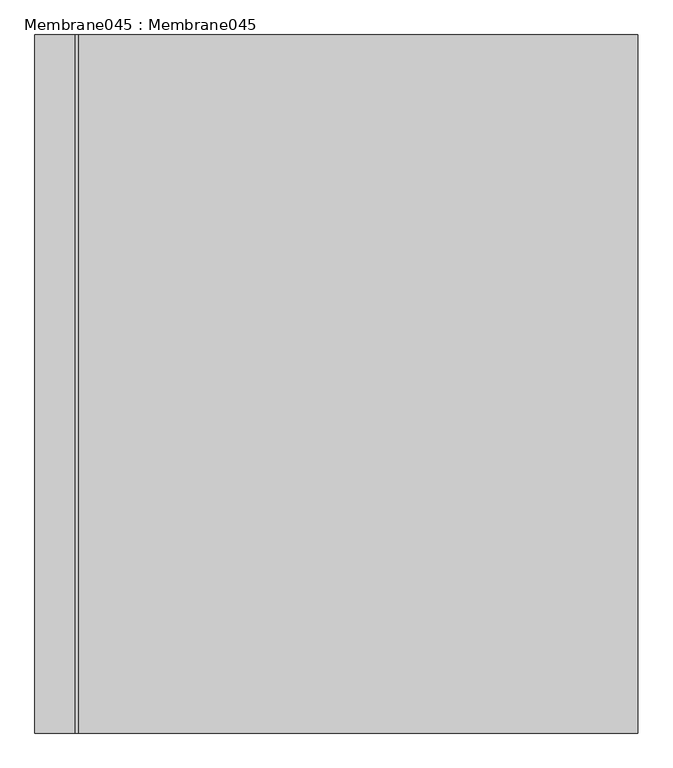
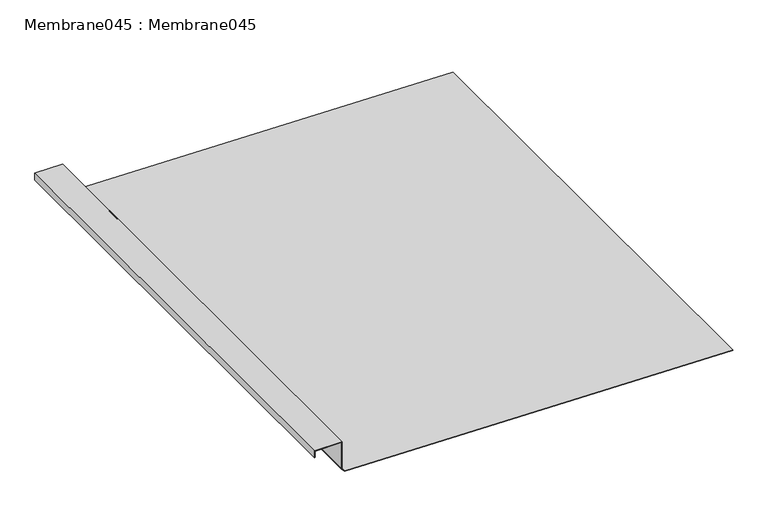
"""IFC4 building model written with IfcOpenShell, lengths in millimetres: proxy geometry, Membrane045 : Membrane045."""

from ifc_helpers import new_model, si_unit, frame, origin, place, context, project, spatial, polyline, outline, extrude, source, transform, mapped, element, save


def membrane045_membrane045_dc4fe3ef(model_context):
    return source(origin(), model_context, "Body", "SweptSolid", [
        extrude(outline(polyline([(40136.1757812, -7230.3012695), (40136.1757812, -7228.3012695), (40163.4960083, -7228.3012695), (40163.4960083, -7118.3154297), (40045.8515625, -7118.3154297), (40034.453125, -7107.1005859), (40000.937504, -5503.7121051), (40002.9370672, -5503.6703083), (40036.4356875, -7106.2454745), (40046.6704939, -7116.3154297), (40165.4960083, -7116.3154297), (40165.4960083, -7230.3012695), (40136.1757812, -7230.3012695)])), frame((0.0, 7982.1531721, 0.0), z_axis=(0.0, 1.0, 0.0), x_axis=(0.0, 0.0, 1.0)), (0.0, 0.0, 1.0), 2000.0),
    ])


if __name__ == "__main__":
    model = new_model("IFC4")
    model_context = context("Model", 3, world=origin())
    ifc_project = project(units=[si_unit("LENGTHUNIT", "METRE", prefix="MILLI")], contexts=[model_context])
    site = spatial("IfcSite", under=ifc_project)
    building = spatial("IfcBuilding", under=site)
    placement = place(None, origin())
    membrane045_membrane045_shape = membrane045_membrane045_dc4fe3ef(model_context)
    element("IfcBuildingElementProxy", 1, Name="Membrane045 : Membrane045", ObjectType="Membrane045 : Membrane045", at=placement, inside=building, context=model_context, shape_type="MappedRepresentation", body=[
        mapped(membrane045_membrane045_shape, transform((0.0, 0.0, 0.0), x_axis=(1.0, 0.0, 0.0), y_axis=(0.0, 1.0, 0.0), z_axis=(0.0, 0.0, 1.0))),
    ])
    save(model, "model.ifc")

# Revit data of these elements
# Type "Membrane045 : Membrane045"
#   NameOverride = "Membrane045"
# Element 1 (IfcBuildingElementProxy, "Membrane045 : Membrane045")
#   Materials on its faces: "WESTCOAT ALX UNDER TILE WATERPROOFING SYSTEM (FOLLOW MANUFACTURER'S INSTALLATION REQUIREMENTS)"
# Materials
#   "WESTCOAT ALX UNDER TILE WATERPROOFING SYSTEM (FOLLOW MANUFACTURER'S INSTALLATION REQUIREMENTS)": class "Unassigned", colour RGB 179 255 168, transparency 0, Cost = 0
